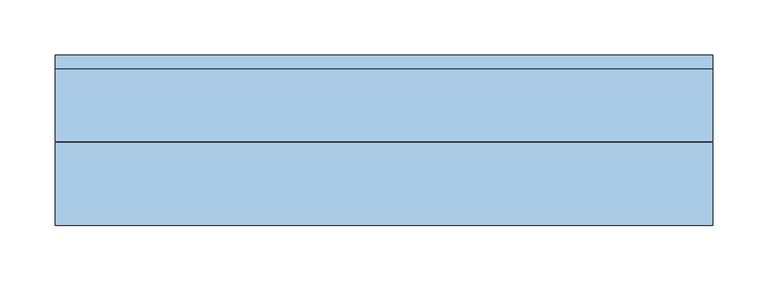
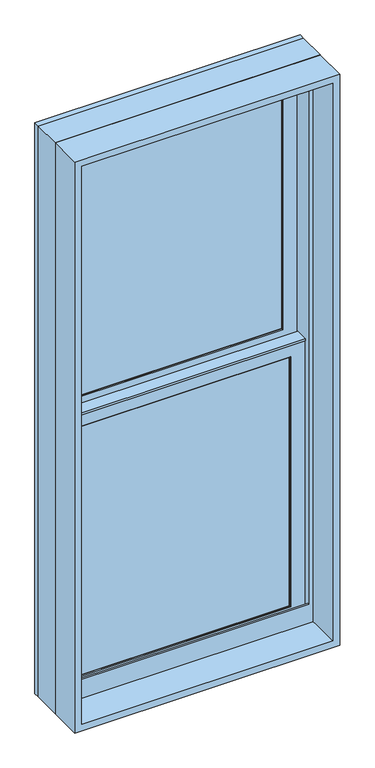
"""IFC4 building model written with IfcOpenShell, lengths in millimetres: window geometry, Window-Double_Hung-Marvin-Essential : ESDH2046."""

from ifc_helpers import new_model, si_unit, frame, origin, place, context, project, spatial, polyline, outline, extrude, faceted_brep, source, transform, mapped, element, save


def window_f747444a(model_context):
    return source(origin(), model_context, "Body", "SolidModel", [
        extrude(outline(polyline([(89.9583333, 20.6375), (89.9583333, 15.875), (70.9083333, 15.875), (70.9083333, 20.6375), (89.9583333, 20.6375)])), frame((0.0, 0.0, 1136.65), z_axis=(0.0, 0.0, 1.0), x_axis=(1.0, 0.0, 0.0)), (0.0, 0.0, 1.0), 603.25),
        extrude(outline(polyline([(-70.9083333, 20.6375), (-70.9083333, 15.875), (-89.9583333, 15.875), (-89.9583333, 20.6375), (-70.9083333, 20.6375)])), frame((0.0, 0.0, 1136.65), z_axis=(0.0, 0.0, 1.0), x_axis=(1.0, 0.0, 0.0)), (0.0, 0.0, 1.0), 603.25),
        extrude(outline(polyline([(241.3, 20.6375), (241.3, 15.875), (-241.3, 15.875), (-241.3, 20.6375), (241.3, 20.6375)])), frame((0.0, 0.0, 1428.75), z_axis=(0.0, 0.0, 1.0), x_axis=(1.0, 0.0, 0.0)), (0.0, 0.0, 1.0), 19.05),
        extrude(outline(polyline([(-89.9583333, 46.83125), (-89.9583333, 51.59375), (-70.9083333, 51.59375), (-70.9083333, 46.83125), (-89.9583333, 46.83125)])), frame((0.0, 0.0, 1778.0), z_axis=(0.0, 0.0, 1.0), x_axis=(1.0, 0.0, 0.0)), (0.0, 0.0, 1.0), 603.25),
        extrude(outline(polyline([(70.9083333, 46.83125), (70.9083333, 51.59375), (89.9583333, 51.59375), (89.9583333, 46.83125), (70.9083333, 46.83125)])), frame((0.0, 0.0, 1778.0), z_axis=(0.0, 0.0, 1.0), x_axis=(1.0, 0.0, 0.0)), (0.0, 0.0, 1.0), 603.25),
        extrude(outline(polyline([(-241.3, 46.83125), (-241.3, 51.59375), (241.3, 51.59375), (241.3, 46.83125), (-241.3, 46.83125)])), frame((0.0, 0.0, 2070.1), z_axis=(0.0, 0.0, 1.0), x_axis=(1.0, 0.0, 0.0)), (0.0, 0.0, 1.0), 19.05),
        extrude(outline(polyline([(89.9583333, 20.6375), (70.9083333, 20.6375), (70.9083333, 25.4), (89.9583333, 25.4), (89.9583333, 20.6375)])), frame((0.0, 0.0, 1136.65), z_axis=(0.0, 0.0, 1.0), x_axis=(1.0, 0.0, 0.0)), (0.0, 0.0, 1.0), 603.25),
        extrude(outline(polyline([(-70.9083333, 20.6375), (-89.9583333, 20.6375), (-89.9583333, 25.4), (-70.9083333, 25.4), (-70.9083333, 20.6375)])), frame((0.0, 0.0, 1136.65), z_axis=(0.0, 0.0, 1.0), x_axis=(1.0, 0.0, 0.0)), (0.0, 0.0, 1.0), 603.25),
        extrude(outline(polyline([(241.3, 20.6375), (-241.3, 20.6375), (-241.3, 25.4), (241.3, 25.4), (241.3, 20.6375)])), frame((0.0, 0.0, 1428.75), z_axis=(0.0, 0.0, 1.0), x_axis=(1.0, 0.0, 0.0)), (0.0, 0.0, 1.0), 19.05),
        extrude(outline(polyline([(-89.9583333, 56.35625), (-70.9083333, 56.35625), (-70.9083333, 51.59375), (-89.9583333, 51.59375), (-89.9583333, 56.35625)])), frame((0.0, 0.0, 1778.0), z_axis=(0.0, 0.0, 1.0), x_axis=(1.0, 0.0, 0.0)), (0.0, 0.0, 1.0), 603.25),
        extrude(outline(polyline([(70.9083333, 56.35625), (89.9583333, 56.35625), (89.9583333, 51.59375), (70.9083333, 51.59375), (70.9083333, 56.35625)])), frame((0.0, 0.0, 1778.0), z_axis=(0.0, 0.0, 1.0), x_axis=(1.0, 0.0, 0.0)), (0.0, 0.0, 1.0), 603.25),
        extrude(outline(polyline([(-241.3, 56.35625), (241.3, 56.35625), (241.3, 51.59375), (-241.3, 51.59375), (-241.3, 56.35625)])), frame((0.0, 0.0, 2070.1), z_axis=(0.0, 0.0, 1.0), x_axis=(1.0, 0.0, 0.0)), (0.0, 0.0, 1.0), 19.05),
        faceted_brep([(-268.2875, 5.6780605, 1769.9351748), (-268.2875, 5.6780605, 1765.3), (268.2875, 5.6780605, 1765.3), (268.2875, 5.6780605, 1769.9351748), (-268.2875, 34.8118605, 1769.9351748), (268.2875, 34.8118605, 1769.9351748), (268.2875, 34.8118605, 1765.3), (-268.2875, 34.8118605, 1765.3), (-268.2875, 30.1625, 1765.3), (-268.2875, 30.1625, 1109.6625), (-268.2875, 8.9241104, 1109.6625), (-268.2875, 8.9241104, 1765.3), (268.2875, 8.9241104, 1765.3), (268.2875, 30.1625, 1765.3), (268.2875, 8.9241104, 1109.6625), (268.2875, 30.1625, 1109.6625), (-252.4034752, 11.90625, 1751.0034752), (-252.4034752, 30.1625, 1751.0034752), (252.4034752, 30.1625, 1751.0034752), (252.4034752, 11.90625, 1751.0034752), (-235.74375, 10.4662439, 1734.34375), (-235.74375, 11.90625, 1734.34375), (235.74375, 11.90625, 1734.34375), (235.74375, 10.4662439, 1734.34375), (237.2858834, 8.9241104, 1735.8858834), (-237.2858834, 8.9241104, 1735.8858834), (252.4034752, 30.1625, 1125.5465248), (252.4034752, 11.90625, 1125.5465248), (235.74375, 11.90625, 1142.20625), (235.74375, 10.4662439, 1142.20625), (237.2858834, 8.9241104, 1140.6641166), (-252.4034752, 30.1625, 1125.5465248), (-252.4034752, 11.90625, 1125.5465248), (-235.74375, 11.90625, 1142.20625), (-235.74375, 10.4662439, 1142.20625), (-237.2858834, 8.9241104, 1140.6641166)], [[[0, 1, 2, 3]], [[4, 5, 6, 7]], [[1, 0, 4, 7, 8, 9, 10, 11]], [[2, 1, 11, 12]], [[7, 6, 13, 8]], [[3, 2, 12, 14, 15, 13, 6, 5]], [[0, 3, 5, 4]], [[16, 17, 18, 19]], [[20, 21, 22, 23]], [[20, 23, 24, 25]], [[19, 18, 26, 27]], [[23, 22, 28, 29]], [[24, 23, 29, 30]], [[27, 26, 31, 32]], [[29, 28, 33, 34]], [[30, 29, 34, 35]], [[15, 14, 10, 9]], [[15, 9, 8, 13], [18, 17, 31, 26]], [[17, 16, 32, 31]], [[16, 19, 27, 32], [22, 21, 33, 28]], [[21, 20, 34, 33]], [[20, 25, 35, 34]], [[10, 14, 12, 11], [25, 24, 30, 35]]]),
        extrude(outline(polyline([(38.5955581, 1751.0125), (33.5778968, 1751.0125), (33.5778968, 1752.6), (39.9405976, 1752.6), (39.9405976, 1751.0125), (61.515625, 1751.0125), (47.6307501, 1747.6975159), (38.5955581, 1747.6975159), (38.5955581, 1751.0125)])), frame((-268.2875, 0.0, 0.0), z_axis=(1.0, 0.0, 0.0), x_axis=(0.0, 1.0, 0.0)), (0.0, 0.0, 1.0), 536.575),
        faceted_brep([(298.45, 0.0, 1079.5), (298.45, 0.0, 2438.4), (-298.45, 0.0, 2438.4), (-298.45, 0.0, 1079.5), (272.25625, 0.0, 1140.61875), (-272.25625, 0.0, 1140.61875), (-272.25625, 0.0, 2412.20625), (272.25625, 0.0, 2412.20625), (272.25625, 3.96875, 1079.5), (-272.25625, 3.96875, 1079.5), (-272.25625, 3.96875, 1140.61875), (272.25625, 3.96875, 1140.61875), (-298.45, 65.6828125, 1079.5), (-272.25625, 65.6828125, 1079.5), (272.25625, 65.6828125, 1079.5), (298.45, 65.6828125, 1079.5), (-298.45, 65.6828125, 2438.4), (298.45, 65.6828125, 2438.4), (272.25625, 65.6828125, 2412.20625), (-272.25625, 65.6828125, 2412.20625)], [[[0, 1, 2, 3], [4, 5, 6, 7]], [[8, 9, 10, 11]], [[5, 4, 11, 10]], [[0, 3, 12, 13, 9, 8, 14, 15]], [[13, 12, 16, 17, 15, 14, 18, 19]], [[13, 19, 6, 5, 10, 9]], [[7, 6, 19, 18]], [[18, 14, 8, 11, 4, 7]], [[1, 0, 15, 17]], [[2, 1, 17, 16]], [[3, 2, 16, 12]]]),
        faceted_brep([(272.25625, 30.1625, 1758.95), (270.66875, 30.1625, 1758.95), (270.66875, 30.1625, 1103.8544613), (272.25625, 30.1625, 1103.8544613), (-270.66875, 30.1625, 1758.95), (-272.25625, 30.1625, 1758.95), (-272.25625, 30.1625, 1103.8544613), (-270.66875, 30.1625, 1103.8544613), (270.66875, 63.5, 1758.95), (272.25625, 63.5, 1758.95), (272.25625, 63.5, 1097.3743077), (270.66875, 63.5, 1097.3743077), (-272.25625, 63.5, 1758.95), (-270.66875, 63.5, 1758.95), (-270.66875, 63.5, 1097.3743077), (-272.25625, 63.5, 1097.3743077), (283.5108932, 3.96875, 1108.9460105), (283.5108932, 3.96875, 1079.5), (283.5108932, 65.6828125, 1079.5), (283.5108932, 65.6828125, 1096.950012), (-283.5108932, 3.96875, 1079.5), (-283.5108932, 3.96875, 1108.9460105), (-283.5108932, 65.6828125, 1096.950012), (-283.5108932, 65.6828125, 1079.5), (283.5108932, 78.58125, 1094.4428097), (-283.5108932, 78.58125, 1094.4428097), (-281.4971252, 68.2348864, 1096.4539391), (-263.53135, 68.2348864, 1096.4539391), (-263.53135, 65.6828125, 1096.950012), (263.53135, 65.6828125, 1096.950012), (263.53135, 68.2348864, 1096.4539391), (281.4971252, 68.2348864, 1096.4539391), (-298.45, 65.6828125, 1079.5), (-298.45, 78.5948249, 1079.5), (298.45, 78.5948249, 1079.5), (298.45, 65.6828125, 1079.5), (-298.45, 78.58125, 2438.4), (298.45, 78.58125, 2438.4), (283.5108932, 78.58125, 2423.4608932), (-283.5108932, 78.58125, 2423.4608932), (-298.45, 65.6828125, 2438.4), (-281.4971252, 68.2348864, 2421.4471252), (281.4971252, 68.2348864, 2421.4471252), (263.53135, 68.2348864, 2403.48135), (-263.53135, 68.2348864, 2403.48135), (-263.53135, 65.6828125, 2403.48135), (263.53135, 65.6828125, 2403.48135), (298.45, 65.6828125, 2438.4)], [[[0, 1, 2, 3]], [[4, 5, 6, 7]], [[8, 9, 10, 11]], [[12, 13, 14, 15]], [[1, 8, 11, 2]], [[9, 0, 3, 10]], [[1, 0, 9, 8]], [[5, 4, 13, 12]], [[5, 12, 15, 6]], [[13, 4, 7, 14]], [[16, 17, 18, 19]], [[20, 21, 22, 23]], [[24, 25, 26, 27, 28, 22, 21, 16, 19, 29, 30, 31], [3, 2, 11, 10], [7, 6, 15, 14]], [[17, 16, 21, 20]], [[17, 20, 23, 32, 33, 34, 35, 18]], [[34, 33, 36, 37], [25, 24, 38, 39]], [[33, 32, 40, 36]], [[39, 41, 26, 25]], [[41, 42, 31, 30, 43, 44, 27, 26]], [[44, 45, 28, 27]], [[40, 32, 23, 22, 28, 45, 46, 29, 19, 18, 35, 47]], [[36, 40, 47, 37]], [[39, 38, 42, 41]], [[44, 43, 46, 45]], [[34, 37, 47, 35]], [[42, 38, 24, 31]], [[46, 43, 30, 29]]]),
        extrude(outline(polyline([(248.44375, 11.90625), (-248.44375, 11.90625), (-248.44375, 15.08125), (248.44375, 15.08125), (248.44375, 11.90625)])), frame((0.0, 0.0, 1129.50625), z_axis=(0.0, 0.0, 1.0), x_axis=(1.0, 0.0, 0.0)), (0.0, 0.0, 1.0), 617.5375),
        extrude(outline(polyline([(248.44375, 42.8625), (-248.44375, 42.8625), (-248.44375, 46.0375), (248.44375, 46.0375), (248.44375, 42.8625)])), frame((0.0, 0.0, 1770.85625), z_axis=(0.0, 0.0, 1.0), x_axis=(1.0, 0.0, 0.0)), (0.0, 0.0, 1.0), 617.5375),
        faceted_brep([(-235.74375, 31.194477, 1734.34375), (-237.2858834, 32.7366104, 1735.8858834), (237.2858834, 32.7366104, 1735.8858834), (235.74375, 31.194477, 1734.34375), (-235.74375, 30.1625, 1734.34375), (235.74375, 30.1625, 1734.34375), (-268.2875, 32.7366104, 1766.8875), (-268.2875, 30.1625, 1766.8875), (268.2875, 30.1625, 1766.8875), (268.2875, 32.7366104, 1766.8875), (237.2858834, 32.7366104, 1140.6641166), (235.74375, 31.194477, 1142.20625), (235.74375, 30.1625, 1142.20625), (268.2875, 30.1625, 1109.6625), (268.2875, 32.7366104, 1109.6625), (-237.2858834, 32.7366104, 1140.6641166), (-235.74375, 31.194477, 1142.20625), (-235.74375, 30.1625, 1142.20625), (-268.2875, 30.1625, 1109.6625), (-268.2875, 32.7366104, 1109.6625)], [[[0, 1, 2, 3]], [[4, 0, 3, 5]], [[6, 7, 8, 9]], [[3, 2, 10, 11]], [[5, 3, 11, 12]], [[9, 8, 13, 14]], [[11, 10, 15, 16]], [[12, 11, 16, 17]], [[14, 13, 18, 19]], [[9, 14, 19, 6], [1, 15, 10, 2]], [[16, 15, 1, 0]], [[17, 16, 0, 4]], [[7, 18, 13, 8], [5, 12, 17, 4]], [[19, 18, 7, 6]]]),
        faceted_brep([(-252.4034752, 42.8625, 2392.3534752), (-252.4034752, 61.11875, 2392.3534752), (252.4034752, 61.11875, 2392.3534752), (252.4034752, 42.8625, 2392.3534752), (-235.74375, 41.4224939, 2375.69375), (-235.74375, 42.8625, 2375.69375), (235.74375, 42.8625, 2375.69375), (235.74375, 41.4224939, 2375.69375), (-237.2858834, 39.8803604, 2377.2358834), (237.2858834, 39.8803604, 2377.2358834), (-268.2875, 61.11875, 2408.2375), (-268.2875, 39.8803604, 2408.2375), (268.2875, 39.8803604, 2408.2375), (268.2875, 61.11875, 2408.2375), (252.4034752, 61.11875, 1766.8965248), (252.4034752, 42.8625, 1766.8965248), (235.74375, 42.8625, 1783.55625), (235.74375, 41.4224939, 1783.55625), (237.2858834, 39.8803604, 1782.0141166), (268.2875, 39.8803604, 1751.0125), (268.2875, 61.11875, 1751.0125), (-252.4034752, 61.11875, 1766.8965248), (-252.4034752, 42.8625, 1766.8965248), (-235.74375, 42.8625, 1783.55625), (-235.74375, 41.4224939, 1783.55625), (-237.2858834, 39.8803604, 1782.0141166), (-268.2875, 39.8803604, 1751.0125), (-268.2875, 61.11875, 1751.0125)], [[[0, 1, 2, 3]], [[4, 5, 6, 7]], [[8, 4, 7, 9]], [[10, 11, 12, 13]], [[3, 2, 14, 15]], [[7, 6, 16, 17]], [[9, 7, 17, 18]], [[13, 12, 19, 20]], [[15, 14, 21, 22]], [[17, 16, 23, 24]], [[18, 17, 24, 25]], [[20, 19, 26, 27]], [[13, 20, 27, 10], [1, 21, 14, 2]], [[22, 21, 1, 0]], [[3, 15, 22, 0], [5, 23, 16, 6]], [[24, 23, 5, 4]], [[25, 24, 4, 8]], [[11, 26, 19, 12], [9, 18, 25, 8]], [[27, 26, 11, 10]]]),
        faceted_brep([(-268.2875, 61.11875, 1751.0125), (-268.2875, 63.6928604, 1751.0125), (268.2875, 63.6928604, 1751.0125), (268.2875, 61.11875, 1751.0125), (-235.74375, 62.150727, 1783.55625), (-235.74375, 61.11875, 1783.55625), (235.74375, 61.11875, 1783.55625), (235.74375, 62.150727, 1783.55625), (-237.2858834, 63.6928604, 1782.0141166), (237.2858834, 63.6928604, 1782.0141166), (268.2875, 63.6928604, 2408.2375), (268.2875, 61.11875, 2408.2375), (235.74375, 61.11875, 2375.69375), (235.74375, 62.150727, 2375.69375), (237.2858834, 63.6928604, 2377.2358834), (-268.2875, 63.6928604, 2408.2375), (-268.2875, 61.11875, 2408.2375), (-235.74375, 61.11875, 2375.69375), (-235.74375, 62.150727, 2375.69375), (-237.2858834, 63.6928604, 2377.2358834)], [[[0, 1, 2, 3]], [[4, 5, 6, 7]], [[8, 4, 7, 9]], [[3, 2, 10, 11]], [[7, 6, 12, 13]], [[9, 7, 13, 14]], [[11, 10, 15, 16]], [[13, 12, 17, 18]], [[14, 13, 18, 19]], [[16, 15, 1, 0]], [[3, 11, 16, 0], [5, 17, 12, 6]], [[18, 17, 5, 4]], [[19, 18, 4, 8]], [[1, 15, 10, 2], [9, 14, 19, 8]]]),
        extrude(outline(polyline([(248.44375, 26.19375), (-248.44375, 26.19375), (-248.44375, 30.1625), (248.44375, 30.1625), (248.44375, 26.19375)])), frame((0.0, 0.0, 1129.50625), z_axis=(0.0, 0.0, 1.0), x_axis=(1.0, 0.0, 0.0)), (0.0, 0.0, 1.0), 617.5375),
        extrude(outline(polyline([(248.44375, 57.15), (-248.44375, 57.15), (-248.44375, 61.11875), (248.44375, 61.11875), (248.44375, 57.15)])), frame((0.0, 0.0, 1770.85625), z_axis=(0.0, 0.0, 1.0), x_axis=(1.0, 0.0, 0.0)), (0.0, 0.0, 1.0), 617.5375),
        extrude(outline(polyline([(2438.4, 298.45), (2438.4, -298.45), (1079.5, -298.45), (1079.5, 298.45), (2438.4, 298.45)]), holes=[polyline([(2422.525, 282.575), (1095.375, 282.575), (1095.375, -282.575), (2422.525, -282.575), (2422.525, 282.575)])]), frame((0.0, -76.2, 0.0), z_axis=(0.0, 1.0, 0.0), x_axis=(0.0, 0.0, 1.0)), (0.0, 0.0, 1.0), 75.40625),
    ])


if __name__ == "__main__":
    model = new_model("IFC4")
    model_context = context("Model", 3, world=origin())
    ifc_project = project(units=[si_unit("LENGTHUNIT", "METRE", prefix="MILLI")], contexts=[model_context])
    site = spatial("IfcSite", under=ifc_project)
    building = spatial("IfcBuilding", under=site)
    placement = place(None, origin())
    window_shape = window_f747444a(model_context)
    element("IfcWindow", 1, ObjectType="Window-Double_Hung-Marvin-Essential : ESDH2046", at=placement, inside=building, context=model_context, shape_type="MappedRepresentation", body=[
        mapped(window_shape, transform((0.0, 0.0, 0.0), x_axis=(1.0, 0.0, 0.0), y_axis=(0.0, 1.0, 0.0), z_axis=(0.0, 0.0, 1.0))),
    ])
    save(model, "model.ifc")

# Revit data of these elements
# Type "Window-Double_Hung-Marvin-Essential : ESDH2046"
#   Type Mark = "55"
#   Window Type = "Essential Double Hung"
#   Product data url = "https://bimobject.com/marvin-windows-and-doors/product/marvin-dhwau"
#   Product Guid = "c4a96547-874c-4385-91dc-a058adc19d98"
#   Frame = "All Ultrex"
#   Egress Window = "No"
#   URL = "www.marvin.com"
#   Model = "ESDH2046"
#   Manufacturer = "Marvin Windows and Doors"
#   Label Egress = ""
#   Glass Type = "IG Low E II with Argon"
#   Design Pressure = "DP50"
#   Description = "2454 DBHG"
#   Analytic Construction = "<None>"
#   Prairie Corner Width = 0' - 4"
#   Prairie Corner Height = 0' - 4"
#   Egress Width = 1' - 8 9/16"
#   Egress Height = 1' - 10 27/128"
#   Rough Width = 2' - 0"
#   Rough Height = 4' - 6"
#   Nominal Width = 2' - 0"
#   Nominal Height = 4' - 6"
#   Inset to Installation Flange [instance default] = 0' - 1"
#   Height = 4' - 5 1/2"
#   Egress Area = 3.17161 SF
#   Default Head Height = 8' - 0"
#   Width = 1' - 11 1/2"
#   Daylight Area = 6.01025 SF
#   DLO Width = 1' - 6 9/16"
#   DLO Height = 1' - 11 5/16"
#   Muntins Top Sash = yes
#   Lites Wide Top Sash = 3
#   Lites Wide Bottom Sash = 3
#   Lites High Top Sash = 2
#   Lites High Bottom Sash = 2
#   Lite Cut Prairie 9 = no
#   Lite Cut HV Grid = yes
#   Muntins Bottom Sash = yes
#   Label Visibility = no
#   Jamb Extension Visibility = yes
#   Edition number = 1
#   Interior Material = Ultrex-Marvin-Stonewhite
#   Glazing Material = Glass-Marvin-IG Low E II with Argon
#   Cladding Material = Ultrex-Marvin-Pebblegray
#   Wall Closure = (empty or 0)
#   Assembly Code = ""
# Element 1 (IfcWindow, "Window-Double_Hung-Marvin-Essential : ESDH2046")
#   Materials on its faces: "Ultrex-Marvin-Pebblegray", "Ultrex-Marvin-Stonewhite", "Glass-Marvin-IG Low E II with Argon"
# Materials
#   "Ultrex-Marvin-Stonewhite": class "Paint", colour RGB 250 251 245, transparency 0
#   "Glass-Marvin-IG Low E II with Argon": class "Glass", colour RGB 0 128 192, transparency 0.85
#   "Ultrex-Marvin-Pebblegray": class "Paint", colour RGB 189 185 173, transparency 0
